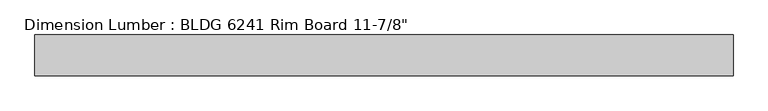
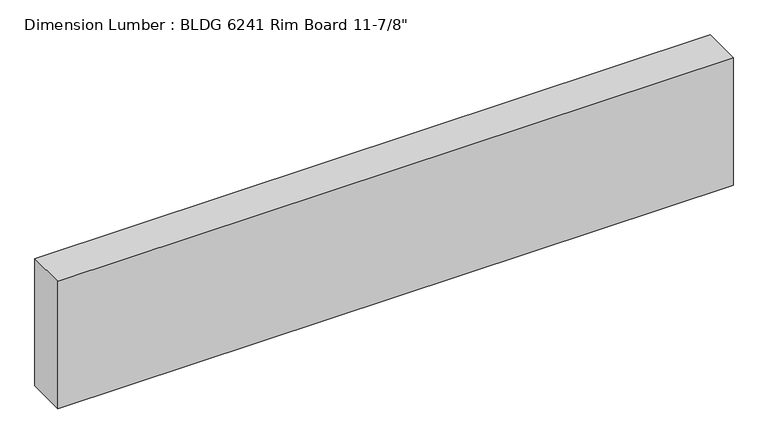
"""IFC4 building model written with IfcOpenShell, lengths in millimetres: beam geometry."""

from ifc_helpers import new_model, si_unit, frame, origin, place, context, project, spatial, polyline, outline, extrude, source, transform, mapped, element, save


def beam_585373de(model_context):
    return source(origin(), model_context, "Body", "SweptSolid", [
        extrude(outline(polyline([(755.65, 44.45), (755.65, -44.45), (-755.65, -44.45), (-755.65, 44.45), (755.65, 44.45)])), frame((0.0, 0.0, -150.8125), z_axis=(0.0, 0.0, 1.0), x_axis=(1.0, 0.0, 0.0)), (0.0, 0.0, 1.0), 301.625),
    ])


if __name__ == "__main__":
    model = new_model("IFC4")
    model_context = context("Model", 3, world=origin())
    ifc_project = project(units=[si_unit("LENGTHUNIT", "METRE", prefix="MILLI")], contexts=[model_context])
    site = spatial("IfcSite", under=ifc_project)
    building = spatial("IfcBuilding", under=site)
    placement = place(None, origin())
    beam_shape = beam_585373de(model_context)
    element("IfcBeam", 1, ObjectType="Dimension Lumber : BLDG 6241 Rim Board 11-7/8\"", at=placement, inside=building, context=model_context, shape_type="MappedRepresentation", body=[
        mapped(beam_shape, transform((0.0, 0.0, 0.0), x_axis=(1.0, 0.0, 0.0), y_axis=(0.0, 1.0, 0.0), z_axis=(0.0, 0.0, 1.0))),
    ])
    save(model, "model.ifc")

# Revit data of these elements
# Type "Dimension Lumber : BLDG 6241 Rim Board 11-7/8\""
#   Assembly Code = "B10"
#   A = 0.273472 SF
#   Length [instance default] = 5' - 0"
#   b = 0' - 3 1/2"
#   d = 0' - 11 7/8"
#   Structural Material [instance default] = Softwood, Lumber
# Element 1 (IfcBeam, "Dimension Lumber : BLDG 6241 Rim Board 11-7/8\"")
#   Materials on its faces: "Softwood, Lumber"
# Materials
#   "Softwood, Lumber": class "Wood", colour RGB 223 192 134, transparency 0, Description = "Pinus Echinata", Cost = 0
